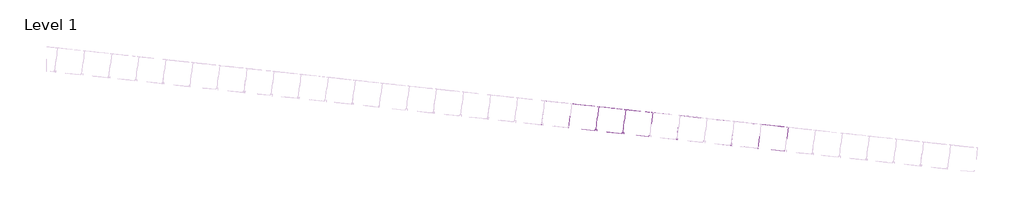
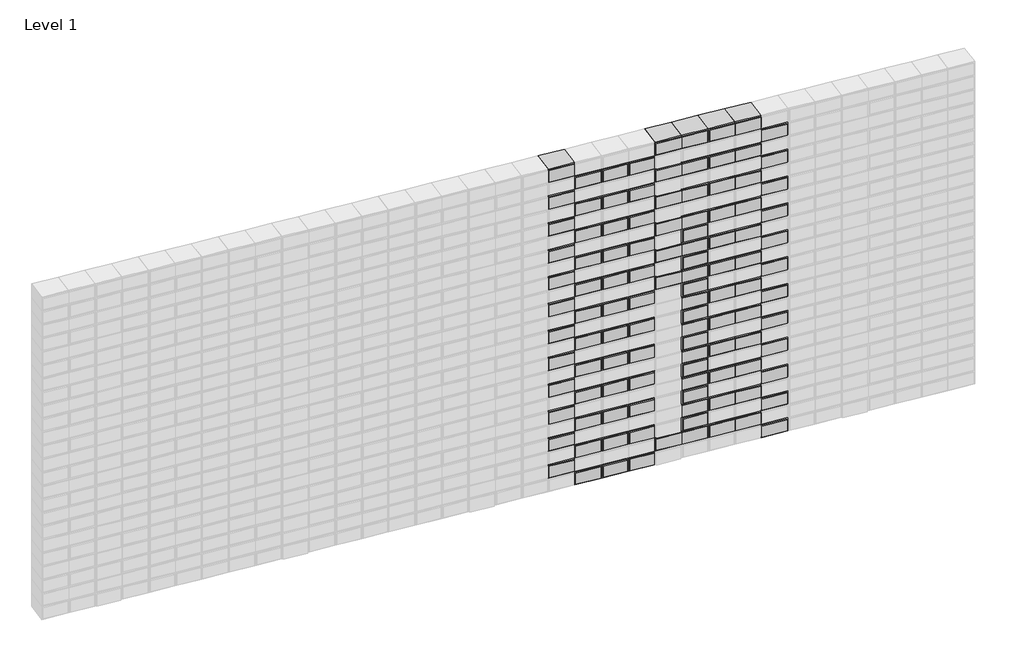
# One storey, part 16 of 18: 111 proxies.
"""IFC4 building model written with IfcOpenShell, lengths in millimetres."""

import ifcopenshell
import ifcopenshell.guid

model = None  # the IFC model being written
_history = None  # IfcOwnerHistory: only IFC2X3 demands one
_inside = {}  # id of a spatial element -> (the spatial element, [elements in it])
_under = {}  # id of a project, library or spatial element -> (it, [spatial elements below it])
_declared = {}  # id of a project -> (the project, [libraries it declares])
_typed = {}  # id of a type object -> (the type object, [elements of that type])
_made_of = {}  # id of a material, layer set ... -> (it, [elements and type objects made of it])


def new_model(schema):
    """Start an empty IFC model of exactly this schema.

    Asked for "IFC4X3", IfcOpenShell would pick the latest addendum, in which some entities
    have other attributes; the version numbers below select the first issue.
    IFC2X3 requires an IfcOwnerHistory on every rooted entity: one is made here for all.
    """
    global model, _history
    if schema == "IFC4X3":
        model = ifcopenshell.file(schema_version=(4, 3, 0, 0))
    else:
        model = ifcopenshell.file(schema=schema)
    _inside.clear()
    _under.clear()
    _declared.clear()
    _typed.clear()
    _made_of.clear()
    _history = None
    if model.schema == "IFC2X3":
        org = make("IfcOrganization", Name="unknown")
        user = make(
            "IfcPersonAndOrganization",
            ThePerson=make("IfcPerson", FamilyName="unknown"),
            TheOrganization=org,
        )
        app = make(
            "IfcApplication",
            ApplicationDeveloper=org,
            Version="unknown",
            ApplicationFullName="unknown",
            ApplicationIdentifier="unknown",
        )
        _history = make(
            "IfcOwnerHistory",
            OwningUser=user,
            OwningApplication=app,
            ChangeAction="ADDED",
            CreationDate=0,
        )
    return model


def make(cls, **values):
    """One entity of the class cls with the attributes given. An attribute that is None is left unset."""
    return model.create_entity(
        cls, **{name: value for name, value in values.items() if value is not None}
    )


def rooted(cls, **values):
    """An entity with a GlobalId (a new one), such as an element, a storey or a relation."""
    return make(cls, GlobalId=ifcopenshell.guid.new(), OwnerHistory=_history, **values)


def si_unit(unit_type, name, prefix=None):
    """IfcSIUnit, for example si_unit("LENGTHUNIT", "METRE", prefix="MILLI")."""
    return make("IfcSIUnit", UnitType=unit_type, Prefix=prefix, Name=name)


def assignment(units):
    """IfcUnitAssignment: the units of a project."""
    return None if units is None else make("IfcUnitAssignment", Units=units)


def point(xyz):
    """IfcCartesianPoint."""
    return None if xyz is None else make("IfcCartesianPoint", Coordinates=xyz)


def direction(xyz):
    """IfcDirection."""
    return None if xyz is None else make("IfcDirection", DirectionRatios=xyz)


def frame(location, z_axis=None, x_axis=None):
    """IfcAxis2Placement3D, a coordinate frame: its origin and axes. An axis left out is left unset."""
    return make(
        "IfcAxis2Placement3D",
        Location=point(location),
        Axis=direction(z_axis),
        RefDirection=direction(x_axis),
    )


def origin():
    """The frame at (0, 0, 0) with its axes left unset."""
    return frame((0.0, 0.0, 0.0))


def origin_with_axes():
    """The frame at (0, 0, 0) with the z axis (0, 0, 1) and the x axis (1, 0, 0) written out."""
    return frame((0.0, 0.0, 0.0), z_axis=(0.0, 0.0, 1.0), x_axis=(1.0, 0.0, 0.0))


def place(relative_to, where):
    """IfcLocalPlacement: puts the frame where relative to a parent placement (None: the world)."""
    return make(
        "IfcLocalPlacement", PlacementRelTo=relative_to, RelativePlacement=where
    )


def context(
    kind, dimensions, precision=None, world=None, true_north=None, identifier=None
):
    """IfcGeometricRepresentationContext, for example the 3D "Model" context."""
    return make(
        "IfcGeometricRepresentationContext",
        ContextIdentifier=identifier,
        ContextType=kind,
        CoordinateSpaceDimension=dimensions,
        Precision=precision,
        WorldCoordinateSystem=world,
        TrueNorth=true_north,
    )


def project(units=None, contexts=None):
    """IfcProject with its units and contexts."""
    return rooted(
        "IfcProject",
        Name="project",
        RepresentationContexts=contexts,
        UnitsInContext=assignment(units),
    )


def spatial(cls, under=None, at=None, **own):
    """A site, building, storey or space (cls), placed at a placement, below another one or the project."""
    s = rooted(cls, ObjectPlacement=at, **own)
    if under is not None:
        _under.setdefault(under.id(), (under, []))[1].append(s)
    return s


def polyline(points):
    """IfcPolyline through the points."""
    return make("IfcPolyline", Points=[point(p) for p in points])


def outline(outer, holes=None, kind="AREA"):
    """IfcArbitraryClosedProfileDef: a profile drawn as a closed curve; with holes, ...WithVoids."""
    if holes is None:
        return make("IfcArbitraryClosedProfileDef", ProfileType=kind, OuterCurve=outer)
    return make(
        "IfcArbitraryProfileDefWithVoids",
        ProfileType=kind,
        OuterCurve=outer,
        InnerCurves=holes,
    )


def extrude(swept, where, along, depth):
    """IfcExtrudedAreaSolid: the profile swept, set in the frame where, extruded along a direction by depth."""
    return make(
        "IfcExtrudedAreaSolid",
        SweptArea=swept,
        Position=where,
        ExtrudedDirection=direction(along),
        Depth=depth,
    )


def shape(context_of_items, identifier, shape_type, items):
    """IfcShapeRepresentation: the items that make up one representation, for example the "Body"."""
    return make(
        "IfcShapeRepresentation",
        ContextOfItems=context_of_items,
        RepresentationIdentifier=identifier,
        RepresentationType=shape_type,
        Items=items,
    )


def source(mapping_origin, context_of_items, identifier, shape_type, items):
    """IfcRepresentationMap: a shape defined once, which mapped items show again and again."""
    return make(
        "IfcRepresentationMap",
        MappingOrigin=mapping_origin,
        MappedRepresentation=shape(context_of_items, identifier, shape_type, items),
    )


def transform(
    local_origin,
    x_axis=None,
    y_axis=None,
    z_axis=None,
    scale=None,
    scale2=None,
    scale3=None,
    uniform=True,
):
    """IfcCartesianTransformationOperator3D, or its non-uniform kind. x_axis, y_axis, z_axis: its Axis1, 2, 3."""
    if uniform:
        return make(
            "IfcCartesianTransformationOperator3D",
            Axis1=direction(x_axis),
            Axis2=direction(y_axis),
            LocalOrigin=point(local_origin),
            Scale=scale,
            Axis3=direction(z_axis),
        )
    return make(
        "IfcCartesianTransformationOperator3DnonUniform",
        Axis1=direction(x_axis),
        Axis2=direction(y_axis),
        LocalOrigin=point(local_origin),
        Scale=scale,
        Axis3=direction(z_axis),
        Scale2=scale2,
        Scale3=scale3,
    )


def mapped(mapping_source, mapping_target):
    """IfcMappedItem: shows the shape of a source again, moved by a transform."""
    return make(
        "IfcMappedItem", MappingSource=mapping_source, MappingTarget=mapping_target
    )


def made_of(thing, what):
    """Note that an element or type object is made of a material, layer set ...; save() writes the relation."""
    if what is not None:
        _made_of.setdefault(what.id(), (what, []))[1].append(thing)
    return thing


def element(
    cls,
    number,
    at=None,
    inside=None,
    cuts=None,
    type_object=None,
    material=None,
    context=None,
    identifier="Body",
    shape_type=None,
    held_by="IfcProductDefinitionShape",
    body=None,
    shapes=None,
    **own,
):
    """One element of the class cls, such as IfcWall. Its Tag is "e" and its number.

    at: its placement. inside: the storey or other place that contains it. cuts: it is an
    opening in that element (IfcRelVoidsElement). A single representation is given by context,
    identifier, shape_type and body (its items); several are given by shapes. held_by: the class
    of the entity that holds the representations. save() writes the other relations.
    """
    e = rooted(cls, Tag="e%d" % number, ObjectPlacement=at, **own)
    if body is not None:
        shapes = [shape(context, identifier, shape_type, body)]
    if shapes is not None:
        e.Representation = make(held_by, Representations=shapes)
    if inside is not None:
        _inside.setdefault(inside.id(), (inside, []))[1].append(e)
    if cuts is not None:
        rooted(
            "IfcRelVoidsElement", RelatingBuildingElement=cuts, RelatedOpeningElement=e
        )
    if type_object is not None:
        _typed.setdefault(type_object.id(), (type_object, []))[1].append(e)
    return made_of(e, material)


def aggregate(whole, parts):
    """IfcRelAggregates: a whole, such as a stair, and the parts it consists of."""
    return rooted("IfcRelAggregates", RelatingObject=whole, RelatedObjects=parts)


def save(model, path):
    """Write the relations noted so far, then the file.

    IfcRelAggregates (storeys below a building ...), IfcRelContainedInSpatialStructure (elements
    in a storey), IfcRelDefinesByType, IfcRelAssociatesMaterial and IfcRelDeclares: one each for
    every whole, place, type object, material and project.
    """
    for whole, parts in _under.values():
        aggregate(whole, parts)
    for where, things in _inside.values():
        rooted(
            "IfcRelContainedInSpatialStructure",
            RelatedElements=things,
            RelatingStructure=where,
        )
    for kind, things in _typed.values():
        rooted("IfcRelDefinesByType", RelatedObjects=things, RelatingType=kind)
    for what, things in _made_of.values():
        rooted("IfcRelAssociatesMaterial", RelatedObjects=things, RelatingMaterial=what)
    for by, libraries in _declared.values():
        rooted("IfcRelDeclares", RelatingContext=by, RelatedDefinitions=libraries)
    model.write(path)


def geel_a5fc7152(model_context):
    return source(origin(), model_context, "Body", "SweptSolid", [
        extrude(outline(polyline([(131.1871262, 51.8695461), (24.8461542, 24.0369432), (23.5801491, 28.8740117), (125.0840527, 55.4406095), (111.9430518, 105.6488784), (10.4391482, 79.0822806), (9.1731432, 83.919349), (115.5141152, 111.7519519), (131.1871262, 51.8695461)])), origin_with_axes(), (0.0, 0.0, 1.0), 95.0),
        extrude(outline(polyline([(111.9430518, 105.6488784), (125.0840527, 55.4406095), (23.5801491, 28.8740117), (10.4391482, 79.0822806), (111.9430518, 105.6488784)])), origin_with_axes(), (0.0, 0.0, 1.0), 100.0),
    ])


def geel_ff5a4212(model_context):
    return source(origin(), model_context, "Body", "SweptSolid", [
        extrude(outline(polyline([(24.8461542, 24.0369432), (9.1731432, 83.919349), (115.5141152, 111.7519519), (116.7801202, 106.9148835), (15.2762167, 80.3482856), (28.4172176, 30.1400167), (129.9211211, 56.7066146), (131.1871262, 51.8695461), (24.8461542, 24.0369432)])), origin_with_axes(), (0.0, 0.0, 1.0), 95.0),
        extrude(outline(polyline([(116.7801202, 106.9148835), (129.9211211, 56.7066146), (28.4172176, 30.1400167), (15.2762167, 80.3482856), (116.7801202, 106.9148835)])), origin_with_axes(), (0.0, 0.0, 1.0), 100.0),
    ])


def rood_14a66368(model_context):
    return source(origin(), model_context, "Body", "SweptSolid", [
        extrude(outline(polyline([(24.8461542, 24.0369432), (9.1731432, 83.919349), (115.5141152, 111.7519519), (131.1871262, 51.8695461), (24.8461542, 24.0369432)]), holes=[polyline([(125.0840527, 55.4406095), (111.9430518, 105.6488784), (15.2762167, 80.3482856), (28.4172176, 30.1400167), (125.0840527, 55.4406095)])]), origin_with_axes(), (0.0, 0.0, 1.0), 95.0),
        extrude(outline(polyline([(111.9430518, 105.6488784), (125.0840527, 55.4406095), (28.4172176, 30.1400167), (15.2762167, 80.3482856), (111.9430518, 105.6488784)])), origin_with_axes(), (0.0, 0.0, 1.0), 100.0),
    ])


model = new_model("IFC4")

# Units and contexts
model_context = context("Model", 3, world=origin())
ifc_project = project(units=[si_unit("LENGTHUNIT", "METRE", prefix="MILLI")], contexts=[model_context])

# Site, building, storey
site = spatial("IfcSite", under=ifc_project)
building = spatial("IfcBuilding", under=site)
storey = spatial("IfcBuildingStorey", under=building, Name="Level 1", Elevation=0.0)

# Proxies
placement = place(None, origin())
geel_shape = geel_a5fc7152(model_context)
element("IfcBuildingElementProxy", 1, Name="Geel", ObjectType="Geel", at=placement, inside=storey, context=model_context, shape_type="MappedRepresentation", body=[
    mapped(geel_shape, transform((11609.0111995, -4573.7784941, 2168.7358475), x_axis=(0.9617275503729374, -0.1047347566147725, -0.25320100633787673), y_axis=(0.25171277368869216, -0.02741220845642974, 0.9674136914420255), z_axis=(-0.10826263628609081, -0.9941223272738551, 0.0))),
])
element("IfcBuildingElementProxy", 2, Name="Geel", ObjectType="Geel", at=placement, inside=storey, context=model_context, shape_type="MappedRepresentation", body=[
    mapped(geel_shape, transform((11609.0111995, -4573.7784941, 2292.5348104), x_axis=(0.9617275503729374, -0.1047347566147725, -0.25320100633787673), y_axis=(0.25171277368869216, -0.02741220845642974, 0.9674136914420255), z_axis=(-0.10826263628609081, -0.9941223272738551, 0.0))),
])
element("IfcBuildingElementProxy", 3, Name="Geel", ObjectType="Geel", at=placement, inside=storey, context=model_context, shape_type="MappedRepresentation", body=[
    mapped(geel_shape, transform((11609.0111995, -4573.7784941, 2416.3337732), x_axis=(0.9617275503729384, -0.1047347566147726, -0.25320100633787307), y_axis=(0.25171277368868855, -0.02741220845642934, 0.9674136914420265), z_axis=(-0.10826263628609081, -0.994122327273855, 0.0))),
])
element("IfcBuildingElementProxy", 4, Name="Geel", ObjectType="Geel", at=placement, inside=storey, context=model_context, shape_type="MappedRepresentation", body=[
    mapped(geel_shape, transform((11609.0111995, -4573.7784941, 2540.132736), x_axis=(0.9617275503729374, -0.1047347566147725, -0.25320100633787673), y_axis=(0.25171277368869216, -0.02741220845642974, 0.9674136914420255), z_axis=(-0.10826263628609081, -0.9941223272738551, 0.0))),
])
element("IfcBuildingElementProxy", 5, Name="Geel", ObjectType="Geel", at=placement, inside=storey, context=model_context, shape_type="MappedRepresentation", body=[
    mapped(geel_shape, transform((11609.0111995, -4573.7784941, 2663.9316989), x_axis=(0.9617275503729374, -0.1047347566147725, -0.25320100633787673), y_axis=(0.25171277368869216, -0.02741220845642974, 0.9674136914420255), z_axis=(-0.10826263628609081, -0.9941223272738551, 0.0))),
])
element("IfcBuildingElementProxy", 6, Name="Geel", ObjectType="Geel", at=placement, inside=storey, context=model_context, shape_type="MappedRepresentation", body=[
    mapped(geel_shape, transform((11609.0111995, -4573.7784941, 2787.7306617), x_axis=(0.9617275503729374, -0.1047347566147725, -0.25320100633787673), y_axis=(0.25171277368869216, -0.02741220845642974, 0.9674136914420255), z_axis=(-0.10826263628609081, -0.9941223272738551, 0.0))),
])
element("IfcBuildingElementProxy", 7, Name="Geel", ObjectType="Geel", at=placement, inside=storey, context=model_context, shape_type="MappedRepresentation", body=[
    mapped(geel_shape, transform((11609.0111995, -4573.7784941, 2911.5296245), x_axis=(0.9617275503729374, -0.1047347566147725, -0.25320100633787673), y_axis=(0.25171277368869216, -0.02741220845642974, 0.9674136914420255), z_axis=(-0.10826263628609081, -0.9941223272738551, 0.0))),
])
element("IfcBuildingElementProxy", 8, Name="Geel", ObjectType="Geel", at=placement, inside=storey, context=model_context, shape_type="MappedRepresentation", body=[
    mapped(geel_shape, transform((11609.0111995, -4573.7784941, 3035.3285874), x_axis=(0.9617275503729374, -0.1047347566147725, -0.25320100633787673), y_axis=(0.25171277368869216, -0.02741220845642974, 0.9674136914420255), z_axis=(-0.10826263628609081, -0.9941223272738551, 0.0))),
])
element("IfcBuildingElementProxy", 9, Name="Geel", ObjectType="Geel", at=placement, inside=storey, context=model_context, shape_type="MappedRepresentation", body=[
    mapped(geel_shape, transform((11609.0111995, -4573.7784941, 3159.1275502), x_axis=(0.9617275503729374, -0.1047347566147725, -0.25320100633787673), y_axis=(0.25171277368869216, -0.02741220845642974, 0.9674136914420255), z_axis=(-0.10826263628609081, -0.9941223272738551, 0.0))),
])
element("IfcBuildingElementProxy", 10, Name="Geel", ObjectType="Geel", at=placement, inside=storey, context=model_context, shape_type="MappedRepresentation", body=[
    mapped(geel_shape, transform((11609.0111995, -4573.7784941, 3282.926513), x_axis=(0.9617275503729374, -0.1047347566147725, -0.25320100633787673), y_axis=(0.25171277368869216, -0.02741220845642974, 0.9674136914420255), z_axis=(-0.10826263628609081, -0.9941223272738551, 0.0))),
])
element("IfcBuildingElementProxy", 11, Name="Geel", ObjectType="Geel", at=placement, inside=storey, context=model_context, shape_type="MappedRepresentation", body=[
    mapped(geel_shape, transform((11609.0111995, -4573.7784941, 3406.7254759), x_axis=(0.9617275503729374, -0.1047347566147725, -0.25320100633787673), y_axis=(0.25171277368869216, -0.02741220845642974, 0.9674136914420255), z_axis=(-0.10826263628609081, -0.9941223272738551, 0.0))),
])
element("IfcBuildingElementProxy", 12, Name="Geel", ObjectType="Geel", at=placement, inside=storey, context=model_context, shape_type="MappedRepresentation", body=[
    mapped(geel_shape, transform((11609.0111995, -4573.7784941, 2044.9368847), x_axis=(0.9617275503729384, -0.1047347566147726, -0.25320100633787307), y_axis=(0.25171277368868855, -0.02741220845642934, 0.9674136914420265), z_axis=(-0.10826263628609081, -0.994122327273855, 0.0))),
])
element("IfcBuildingElementProxy", 13, Name="Geel", ObjectType="Geel", at=placement, inside=storey, context=model_context, shape_type="MappedRepresentation", body=[
    mapped(geel_shape, transform((11062.6268786, -4514.2757494, 2168.7358475), x_axis=(0.9617275503729374, -0.1047347566147725, -0.25320100633787673), y_axis=(0.25171277368869216, -0.02741220845642974, 0.9674136914420255), z_axis=(-0.10826263628609081, -0.9941223272738551, 0.0))),
])
element("IfcBuildingElementProxy", 14, Name="Geel", ObjectType="Geel", at=placement, inside=storey, context=model_context, shape_type="MappedRepresentation", body=[
    mapped(geel_shape, transform((11827.5649279, -4597.579592, 2168.7358475), x_axis=(0.9617275503729414, -0.10473475661477494, -0.25320100633786047), y_axis=(0.251712773688676, -0.027412208456428513, 0.9674136914420297), z_axis=(-0.10826263628609288, -0.9941223272738549, 0.0))),
])
element("IfcBuildingElementProxy", 15, Name="Geel", ObjectType="Geel", at=placement, inside=storey, context=model_context, shape_type="MappedRepresentation", body=[
    mapped(geel_shape, transform((11062.6268786, -4514.2757494, 2292.5348104), x_axis=(0.9617275503729374, -0.1047347566147725, -0.25320100633787673), y_axis=(0.25171277368869216, -0.02741220845642974, 0.9674136914420255), z_axis=(-0.10826263628609081, -0.9941223272738551, 0.0))),
])
element("IfcBuildingElementProxy", 16, Name="Geel", ObjectType="Geel", at=placement, inside=storey, context=model_context, shape_type="MappedRepresentation", body=[
    mapped(geel_shape, transform((11827.5649279, -4597.579592, 2292.5348104), x_axis=(0.9617275503729414, -0.10473475661477494, -0.25320100633786047), y_axis=(0.251712773688676, -0.027412208456428513, 0.9674136914420297), z_axis=(-0.10826263628609288, -0.9941223272738549, 0.0))),
])
element("IfcBuildingElementProxy", 17, Name="Geel", ObjectType="Geel", at=placement, inside=storey, context=model_context, shape_type="MappedRepresentation", body=[
    mapped(geel_shape, transform((11062.6268786, -4514.2757494, 2416.3337732), x_axis=(0.9617275503729384, -0.1047347566147726, -0.25320100633787307), y_axis=(0.25171277368868855, -0.02741220845642934, 0.9674136914420265), z_axis=(-0.10826263628609081, -0.994122327273855, 0.0))),
])
element("IfcBuildingElementProxy", 18, Name="Geel", ObjectType="Geel", at=placement, inside=storey, context=model_context, shape_type="MappedRepresentation", body=[
    mapped(geel_shape, transform((11827.5649279, -4597.579592, 2416.3337732), x_axis=(0.9617275503729424, -0.10473475661477503, -0.25320100633785697), y_axis=(0.25171277368867234, -0.027412208456428104, 0.9674136914420307), z_axis=(-0.10826263628609285, -0.9941223272738547, 0.0))),
])
element("IfcBuildingElementProxy", 19, Name="Geel", ObjectType="Geel", at=placement, inside=storey, context=model_context, shape_type="MappedRepresentation", body=[
    mapped(geel_shape, transform((11062.6268786, -4514.2757494, 2540.132736), x_axis=(0.9617275503729374, -0.1047347566147725, -0.25320100633787673), y_axis=(0.25171277368869216, -0.02741220845642974, 0.9674136914420255), z_axis=(-0.10826263628609081, -0.9941223272738551, 0.0))),
])
element("IfcBuildingElementProxy", 20, Name="Geel", ObjectType="Geel", at=placement, inside=storey, context=model_context, shape_type="MappedRepresentation", body=[
    mapped(geel_shape, transform((11827.5649279, -4597.579592, 2540.132736), x_axis=(0.9617275503729414, -0.10473475661477494, -0.25320100633786047), y_axis=(0.251712773688676, -0.027412208456428513, 0.9674136914420297), z_axis=(-0.10826263628609288, -0.9941223272738549, 0.0))),
])
element("IfcBuildingElementProxy", 21, Name="Geel", ObjectType="Geel", at=placement, inside=storey, context=model_context, shape_type="MappedRepresentation", body=[
    mapped(geel_shape, transform((11062.6268786, -4514.2757494, 2663.9316989), x_axis=(0.9617275503729374, -0.1047347566147725, -0.25320100633787673), y_axis=(0.25171277368869216, -0.02741220845642974, 0.9674136914420255), z_axis=(-0.10826263628609081, -0.9941223272738551, 0.0))),
])
element("IfcBuildingElementProxy", 22, Name="Geel", ObjectType="Geel", at=placement, inside=storey, context=model_context, shape_type="MappedRepresentation", body=[
    mapped(geel_shape, transform((11827.5649279, -4597.579592, 2663.9316989), x_axis=(0.9617275503729414, -0.10473475661477494, -0.25320100633786047), y_axis=(0.251712773688676, -0.027412208456428513, 0.9674136914420297), z_axis=(-0.10826263628609288, -0.9941223272738549, 0.0))),
])
element("IfcBuildingElementProxy", 23, Name="Geel", ObjectType="Geel", at=placement, inside=storey, context=model_context, shape_type="MappedRepresentation", body=[
    mapped(geel_shape, transform((11062.6268786, -4514.2757494, 2787.7306617), x_axis=(0.9617275503729374, -0.1047347566147725, -0.25320100633787673), y_axis=(0.25171277368869216, -0.02741220845642974, 0.9674136914420255), z_axis=(-0.10826263628609081, -0.9941223272738551, 0.0))),
])
element("IfcBuildingElementProxy", 24, Name="Geel", ObjectType="Geel", at=placement, inside=storey, context=model_context, shape_type="MappedRepresentation", body=[
    mapped(geel_shape, transform((11827.5649279, -4597.579592, 2787.7306617), x_axis=(0.9617275503729414, -0.10473475661477494, -0.25320100633786047), y_axis=(0.251712773688676, -0.027412208456428513, 0.9674136914420297), z_axis=(-0.10826263628609288, -0.9941223272738549, 0.0))),
])
element("IfcBuildingElementProxy", 25, Name="Geel", ObjectType="Geel", at=placement, inside=storey, context=model_context, shape_type="MappedRepresentation", body=[
    mapped(geel_shape, transform((11062.6268786, -4514.2757494, 2911.5296245), x_axis=(0.9617275503729374, -0.1047347566147725, -0.25320100633787673), y_axis=(0.25171277368869216, -0.02741220845642974, 0.9674136914420255), z_axis=(-0.10826263628609081, -0.9941223272738551, 0.0))),
])
element("IfcBuildingElementProxy", 26, Name="Geel", ObjectType="Geel", at=placement, inside=storey, context=model_context, shape_type="MappedRepresentation", body=[
    mapped(geel_shape, transform((11827.5649279, -4597.579592, 2911.5296245), x_axis=(0.9617275503729414, -0.10473475661477494, -0.25320100633786047), y_axis=(0.251712773688676, -0.027412208456428513, 0.9674136914420297), z_axis=(-0.10826263628609288, -0.9941223272738549, 0.0))),
])
element("IfcBuildingElementProxy", 27, Name="Geel", ObjectType="Geel", at=placement, inside=storey, context=model_context, shape_type="MappedRepresentation", body=[
    mapped(geel_shape, transform((11062.6268786, -4514.2757494, 3035.3285874), x_axis=(0.9617275503729374, -0.1047347566147725, -0.25320100633787673), y_axis=(0.25171277368869216, -0.02741220845642974, 0.9674136914420255), z_axis=(-0.10826263628609081, -0.9941223272738551, 0.0))),
])
element("IfcBuildingElementProxy", 28, Name="Geel", ObjectType="Geel", at=placement, inside=storey, context=model_context, shape_type="MappedRepresentation", body=[
    mapped(geel_shape, transform((11827.5649279, -4597.579592, 3035.3285874), x_axis=(0.9617275503729414, -0.10473475661477494, -0.25320100633786047), y_axis=(0.251712773688676, -0.027412208456428513, 0.9674136914420297), z_axis=(-0.10826263628609288, -0.9941223272738549, 0.0))),
])
element("IfcBuildingElementProxy", 29, Name="Geel", ObjectType="Geel", at=placement, inside=storey, context=model_context, shape_type="MappedRepresentation", body=[
    mapped(geel_shape, transform((11062.6268786, -4514.2757494, 3159.1275502), x_axis=(0.9617275503729374, -0.1047347566147725, -0.25320100633787673), y_axis=(0.25171277368869216, -0.02741220845642974, 0.9674136914420255), z_axis=(-0.10826263628609081, -0.9941223272738551, 0.0))),
])
element("IfcBuildingElementProxy", 30, Name="Geel", ObjectType="Geel", at=placement, inside=storey, context=model_context, shape_type="MappedRepresentation", body=[
    mapped(geel_shape, transform((11827.5649279, -4597.579592, 3159.1275502), x_axis=(0.9617275503729414, -0.10473475661477494, -0.25320100633786047), y_axis=(0.251712773688676, -0.027412208456428513, 0.9674136914420297), z_axis=(-0.10826263628609288, -0.9941223272738549, 0.0))),
])
element("IfcBuildingElementProxy", 31, Name="Geel", ObjectType="Geel", at=placement, inside=storey, context=model_context, shape_type="MappedRepresentation", body=[
    mapped(geel_shape, transform((11062.6268786, -4514.2757494, 3282.926513), x_axis=(0.9617275503729374, -0.1047347566147725, -0.25320100633787673), y_axis=(0.25171277368869216, -0.02741220845642974, 0.9674136914420255), z_axis=(-0.10826263628609081, -0.9941223272738551, 0.0))),
])
element("IfcBuildingElementProxy", 32, Name="Geel", ObjectType="Geel", at=placement, inside=storey, context=model_context, shape_type="MappedRepresentation", body=[
    mapped(geel_shape, transform((11827.5649279, -4597.579592, 3282.926513), x_axis=(0.9617275503729414, -0.10473475661477494, -0.25320100633786047), y_axis=(0.251712773688676, -0.027412208456428513, 0.9674136914420297), z_axis=(-0.10826263628609288, -0.9941223272738549, 0.0))),
])
element("IfcBuildingElementProxy", 33, Name="Geel", ObjectType="Geel", at=placement, inside=storey, context=model_context, shape_type="MappedRepresentation", body=[
    mapped(geel_shape, transform((11062.6268786, -4514.2757494, 3406.7254759), x_axis=(0.9617275503729374, -0.1047347566147725, -0.25320100633787673), y_axis=(0.25171277368869216, -0.02741220845642974, 0.9674136914420255), z_axis=(-0.10826263628609081, -0.9941223272738551, 0.0))),
])
element("IfcBuildingElementProxy", 34, Name="Geel", ObjectType="Geel", at=placement, inside=storey, context=model_context, shape_type="MappedRepresentation", body=[
    mapped(geel_shape, transform((11827.5649279, -4597.579592, 3406.7254759), x_axis=(0.9617275503729414, -0.10473475661477494, -0.25320100633786047), y_axis=(0.251712773688676, -0.027412208456428513, 0.9674136914420297), z_axis=(-0.10826263628609288, -0.9941223272738549, 0.0))),
])
element("IfcBuildingElementProxy", 35, Name="Geel", ObjectType="Geel", at=placement, inside=storey, context=model_context, shape_type="MappedRepresentation", body=[
    mapped(geel_shape, transform((11062.6268786, -4514.2757494, 2044.9368847), x_axis=(0.9617275503729384, -0.1047347566147726, -0.25320100633787307), y_axis=(0.25171277368868855, -0.02741220845642934, 0.9674136914420265), z_axis=(-0.10826263628609081, -0.994122327273855, 0.0))),
])
element("IfcBuildingElementProxy", 36, Name="Geel", ObjectType="Geel", at=placement, inside=storey, context=model_context, shape_type="MappedRepresentation", body=[
    mapped(geel_shape, transform((11827.5649279, -4597.579592, 2044.9368847), x_axis=(0.9617275503729424, -0.10473475661477503, -0.25320100633785697), y_axis=(0.25171277368867234, -0.027412208456428104, 0.9674136914420307), z_axis=(-0.10826263628609285, -0.9941223272738547, 0.0))),
])
geel_2_shape = geel_ff5a4212(model_context)
element("IfcBuildingElementProxy", 37, Name="Geel", ObjectType="Geel", at=placement, inside=storey, context=model_context, shape_type="MappedRepresentation", body=[
    mapped(geel_2_shape, transform((11499.7343354, -4561.8779452, 2787.7306617), x_axis=(0.9617275503729381, -0.10473475661476775, -0.25320100633787634), y_axis=(0.2517127736886919, -0.02741220845642843, 0.9674136914420257), z_axis=(-0.1082626362860859, -0.9941223272738555, 0.0))),
])
element("IfcBuildingElementProxy", 38, Name="Geel", ObjectType="Geel", at=placement, inside=storey, context=model_context, shape_type="MappedRepresentation", body=[
    mapped(geel_2_shape, transform((11499.7343354, -4561.8779452, 2911.5296245), x_axis=(0.9617275503729381, -0.10473475661476775, -0.25320100633787634), y_axis=(0.2517127736886919, -0.02741220845642843, 0.9674136914420257), z_axis=(-0.1082626362860859, -0.9941223272738555, 0.0))),
])
element("IfcBuildingElementProxy", 39, Name="Geel", ObjectType="Geel", at=placement, inside=storey, context=model_context, shape_type="MappedRepresentation", body=[
    mapped(geel_2_shape, transform((11499.7343354, -4561.8779452, 3035.3285874), x_axis=(0.9617275503729381, -0.10473475661476775, -0.25320100633787634), y_axis=(0.2517127736886919, -0.02741220845642843, 0.9674136914420257), z_axis=(-0.1082626362860859, -0.9941223272738555, 0.0))),
])
element("IfcBuildingElementProxy", 40, Name="Geel", ObjectType="Geel", at=placement, inside=storey, context=model_context, shape_type="MappedRepresentation", body=[
    mapped(geel_2_shape, transform((11499.7343354, -4561.8779452, 3159.1275502), x_axis=(0.9617275503729381, -0.10473475661476775, -0.25320100633787634), y_axis=(0.2517127736886919, -0.02741220845642843, 0.9674136914420257), z_axis=(-0.1082626362860859, -0.9941223272738555, 0.0))),
])
element("IfcBuildingElementProxy", 41, Name="Geel", ObjectType="Geel", at=placement, inside=storey, context=model_context, shape_type="MappedRepresentation", body=[
    mapped(geel_2_shape, transform((11499.7343354, -4561.8779452, 3282.926513), x_axis=(0.9617275503729381, -0.10473475661476775, -0.25320100633787634), y_axis=(0.2517127736886919, -0.02741220845642843, 0.9674136914420257), z_axis=(-0.1082626362860859, -0.9941223272738555, 0.0))),
])
element("IfcBuildingElementProxy", 42, Name="Geel", ObjectType="Geel", at=placement, inside=storey, context=model_context, shape_type="MappedRepresentation", body=[
    mapped(geel_2_shape, transform((11499.7343354, -4561.8779452, 3406.7254759), x_axis=(0.9617275503729381, -0.10473475661476775, -0.25320100633787634), y_axis=(0.2517127736886919, -0.02741220845642843, 0.9674136914420257), z_axis=(-0.1082626362860859, -0.9941223272738555, 0.0))),
])
element("IfcBuildingElementProxy", 43, Name="Geel", ObjectType="Geel", at=placement, inside=storey, context=model_context, shape_type="MappedRepresentation", body=[
    mapped(geel_2_shape, transform((11499.7343354, -4561.8779452, 2044.9368847), x_axis=(0.961727550372939, -0.10473475661476785, -0.2532010063378727), y_axis=(0.2517127736886882, -0.02741220845642804, 0.9674136914420266), z_axis=(-0.1082626362860859, -0.9941223272738555, 0.0))),
])
element("IfcBuildingElementProxy", 44, Name="Geel", ObjectType="Geel", at=placement, inside=storey, context=model_context, shape_type="MappedRepresentation", body=[
    mapped(geel_2_shape, transform((11718.2880637, -4585.679043, 2168.7358475), x_axis=(0.9617275503729374, -0.1047347566147725, -0.25320100633787673), y_axis=(0.25171277368869216, -0.02741220845642974, 0.9674136914420255), z_axis=(-0.10826263628609081, -0.9941223272738551, 0.0))),
])
element("IfcBuildingElementProxy", 45, Name="Geel", ObjectType="Geel", at=placement, inside=storey, context=model_context, shape_type="MappedRepresentation", body=[
    mapped(geel_2_shape, transform((11718.2880637, -4585.679043, 2292.5348104), x_axis=(0.9617275503729374, -0.1047347566147725, -0.25320100633787673), y_axis=(0.25171277368869216, -0.02741220845642974, 0.9674136914420255), z_axis=(-0.10826263628609081, -0.9941223272738551, 0.0))),
])
element("IfcBuildingElementProxy", 46, Name="Geel", ObjectType="Geel", at=placement, inside=storey, context=model_context, shape_type="MappedRepresentation", body=[
    mapped(geel_2_shape, transform((11718.2880637, -4585.679043, 2416.3337732), x_axis=(0.9617275503729384, -0.1047347566147726, -0.25320100633787307), y_axis=(0.25171277368868855, -0.02741220845642934, 0.9674136914420265), z_axis=(-0.10826263628609081, -0.994122327273855, 0.0))),
])
element("IfcBuildingElementProxy", 47, Name="Geel", ObjectType="Geel", at=placement, inside=storey, context=model_context, shape_type="MappedRepresentation", body=[
    mapped(geel_2_shape, transform((11718.2880637, -4585.679043, 2540.132736), x_axis=(0.9617275503729374, -0.1047347566147725, -0.25320100633787673), y_axis=(0.25171277368869216, -0.02741220845642974, 0.9674136914420255), z_axis=(-0.10826263628609081, -0.9941223272738551, 0.0))),
])
element("IfcBuildingElementProxy", 48, Name="Geel", ObjectType="Geel", at=placement, inside=storey, context=model_context, shape_type="MappedRepresentation", body=[
    mapped(geel_2_shape, transform((11718.2880637, -4585.679043, 2663.9316989), x_axis=(0.9617275503729374, -0.1047347566147725, -0.25320100633787673), y_axis=(0.25171277368869216, -0.02741220845642974, 0.9674136914420255), z_axis=(-0.10826263628609081, -0.9941223272738551, 0.0))),
])
element("IfcBuildingElementProxy", 49, Name="Geel", ObjectType="Geel", at=placement, inside=storey, context=model_context, shape_type="MappedRepresentation", body=[
    mapped(geel_2_shape, transform((11718.2880637, -4585.679043, 2787.7306617), x_axis=(0.9617275503729374, -0.1047347566147725, -0.25320100633787673), y_axis=(0.25171277368869216, -0.02741220845642974, 0.9674136914420255), z_axis=(-0.10826263628609081, -0.9941223272738551, 0.0))),
])
element("IfcBuildingElementProxy", 50, Name="Geel", ObjectType="Geel", at=placement, inside=storey, context=model_context, shape_type="MappedRepresentation", body=[
    mapped(geel_2_shape, transform((11718.2880637, -4585.679043, 2911.5296245), x_axis=(0.9617275503729374, -0.1047347566147725, -0.25320100633787673), y_axis=(0.25171277368869216, -0.02741220845642974, 0.9674136914420255), z_axis=(-0.10826263628609081, -0.9941223272738551, 0.0))),
])
element("IfcBuildingElementProxy", 51, Name="Geel", ObjectType="Geel", at=placement, inside=storey, context=model_context, shape_type="MappedRepresentation", body=[
    mapped(geel_2_shape, transform((11718.2880637, -4585.679043, 3035.3285874), x_axis=(0.9617275503729374, -0.1047347566147725, -0.25320100633787673), y_axis=(0.25171277368869216, -0.02741220845642974, 0.9674136914420255), z_axis=(-0.10826263628609081, -0.9941223272738551, 0.0))),
])
element("IfcBuildingElementProxy", 52, Name="Geel", ObjectType="Geel", at=placement, inside=storey, context=model_context, shape_type="MappedRepresentation", body=[
    mapped(geel_2_shape, transform((11718.2880637, -4585.679043, 3159.1275502), x_axis=(0.9617275503729374, -0.1047347566147725, -0.25320100633787673), y_axis=(0.25171277368869216, -0.02741220845642974, 0.9674136914420255), z_axis=(-0.10826263628609081, -0.9941223272738551, 0.0))),
])
element("IfcBuildingElementProxy", 53, Name="Geel", ObjectType="Geel", at=placement, inside=storey, context=model_context, shape_type="MappedRepresentation", body=[
    mapped(geel_2_shape, transform((11718.2880637, -4585.679043, 3282.926513), x_axis=(0.9617275503729374, -0.1047347566147725, -0.25320100633787673), y_axis=(0.25171277368869216, -0.02741220845642974, 0.9674136914420255), z_axis=(-0.10826263628609081, -0.9941223272738551, 0.0))),
])
element("IfcBuildingElementProxy", 54, Name="Geel", ObjectType="Geel", at=placement, inside=storey, context=model_context, shape_type="MappedRepresentation", body=[
    mapped(geel_2_shape, transform((11718.2880637, -4585.679043, 3406.7254759), x_axis=(0.9617275503729374, -0.1047347566147725, -0.25320100633787673), y_axis=(0.25171277368869216, -0.02741220845642974, 0.9674136914420255), z_axis=(-0.10826263628609081, -0.9941223272738551, 0.0))),
])
element("IfcBuildingElementProxy", 55, Name="Geel", ObjectType="Geel", at=placement, inside=storey, context=model_context, shape_type="MappedRepresentation", body=[
    mapped(geel_2_shape, transform((11718.2880637, -4585.679043, 2044.9368847), x_axis=(0.9617275503729384, -0.1047347566147726, -0.25320100633787307), y_axis=(0.25171277368868855, -0.02741220845642934, 0.9674136914420265), z_axis=(-0.10826263628609081, -0.994122327273855, 0.0))),
])
element("IfcBuildingElementProxy", 56, Name="Rood", ObjectType="Rood", at=placement, inside=storey, context=model_context, shape_type="MappedRepresentation", body=[
    mapped(geel_shape, transform((11171.9037428, -4526.1762984, 2106.8363661), x_axis=(0.9617275503729374, -0.1047347566147725, -0.25320100633787673), y_axis=(0.25171277368869216, -0.02741220845642974, 0.9674136914420255), z_axis=(-0.10826263628609081, -0.9941223272738551, 0.0))),
])
element("IfcBuildingElementProxy", 57, Name="Rood", ObjectType="Rood", at=placement, inside=storey, context=model_context, shape_type="MappedRepresentation", body=[
    mapped(geel_shape, transform((11936.8417921, -4609.4801409, 2106.8363661), x_axis=(0.9617275503729374, -0.10473475661477244, -0.25320100633787673), y_axis=(0.25171277368869216, -0.027412208456429728, 0.9674136914420255), z_axis=(-0.10826263628609079, -0.9941223272738551, 0.0))),
])
element("IfcBuildingElementProxy", 58, Name="Rood", ObjectType="Rood", at=placement, inside=storey, context=model_context, shape_type="MappedRepresentation", body=[
    mapped(geel_shape, transform((11171.9037428, -4526.1762984, 2230.6353289), x_axis=(0.9617275503729384, -0.1047347566147726, -0.25320100633787307), y_axis=(0.25171277368868855, -0.02741220845642934, 0.9674136914420265), z_axis=(-0.10826263628609081, -0.994122327273855, 0.0))),
])
element("IfcBuildingElementProxy", 59, Name="Rood", ObjectType="Rood", at=placement, inside=storey, context=model_context, shape_type="MappedRepresentation", body=[
    mapped(geel_shape, transform((11936.8417921, -4609.4801409, 2230.6353289), x_axis=(0.9617275503729384, -0.10473475661477255, -0.25320100633787307), y_axis=(0.25171277368868855, -0.027412208456429325, 0.9674136914420265), z_axis=(-0.10826263628609077, -0.994122327273855, 0.0))),
])
element("IfcBuildingElementProxy", 60, Name="Rood", ObjectType="Rood", at=placement, inside=storey, context=model_context, shape_type="MappedRepresentation", body=[
    mapped(geel_shape, transform((11171.9037428, -4526.1762984, 2354.4342918), x_axis=(0.9617275503729374, -0.1047347566147725, -0.25320100633787673), y_axis=(0.25171277368869216, -0.02741220845642974, 0.9674136914420255), z_axis=(-0.10826263628609081, -0.9941223272738551, 0.0))),
])
element("IfcBuildingElementProxy", 61, Name="Rood", ObjectType="Rood", at=placement, inside=storey, context=model_context, shape_type="MappedRepresentation", body=[
    mapped(geel_shape, transform((11936.8417921, -4609.4801409, 2354.4342918), x_axis=(0.9617275503729374, -0.10473475661477244, -0.25320100633787673), y_axis=(0.25171277368869216, -0.027412208456429728, 0.9674136914420255), z_axis=(-0.10826263628609079, -0.9941223272738551, 0.0))),
])
element("IfcBuildingElementProxy", 62, Name="Rood", ObjectType="Rood", at=placement, inside=storey, context=model_context, shape_type="MappedRepresentation", body=[
    mapped(geel_shape, transform((11171.9037428, -4526.1762984, 2478.2332546), x_axis=(0.9617275503729374, -0.1047347566147725, -0.25320100633787673), y_axis=(0.25171277368869216, -0.02741220845642974, 0.9674136914420255), z_axis=(-0.10826263628609081, -0.9941223272738551, 0.0))),
])
element("IfcBuildingElementProxy", 63, Name="Rood", ObjectType="Rood", at=placement, inside=storey, context=model_context, shape_type="MappedRepresentation", body=[
    mapped(geel_shape, transform((11936.8417921, -4609.4801409, 2478.2332546), x_axis=(0.9617275503729374, -0.10473475661477244, -0.25320100633787673), y_axis=(0.25171277368869216, -0.027412208456429728, 0.9674136914420255), z_axis=(-0.10826263628609079, -0.9941223272738551, 0.0))),
])
element("IfcBuildingElementProxy", 64, Name="Rood", ObjectType="Rood", at=placement, inside=storey, context=model_context, shape_type="MappedRepresentation", body=[
    mapped(geel_shape, transform((11171.9037428, -4526.1762984, 2602.0322174), x_axis=(0.9617275503729394, -0.10473475661477268, -0.2532010063378695), y_axis=(0.2517127736886849, -0.027412208456428923, 0.9674136914420275), z_axis=(-0.1082626362860908, -0.9941223272738551, 0.0))),
])
element("IfcBuildingElementProxy", 65, Name="Rood", ObjectType="Rood", at=placement, inside=storey, context=model_context, shape_type="MappedRepresentation", body=[
    mapped(geel_shape, transform((11936.8417921, -4609.4801409, 2602.0322174), x_axis=(0.9617275503729394, -0.10473475661477262, -0.2532010063378695), y_axis=(0.2517127736886849, -0.027412208456428916, 0.9674136914420275), z_axis=(-0.10826263628609076, -0.9941223272738551, 0.0))),
])
element("IfcBuildingElementProxy", 66, Name="Rood", ObjectType="Rood", at=placement, inside=storey, context=model_context, shape_type="MappedRepresentation", body=[
    mapped(geel_shape, transform((11171.9037428, -4526.1762984, 2725.8311803), x_axis=(0.9617275503729374, -0.1047347566147725, -0.25320100633787673), y_axis=(0.25171277368869216, -0.02741220845642974, 0.9674136914420255), z_axis=(-0.10826263628609081, -0.9941223272738551, 0.0))),
])
element("IfcBuildingElementProxy", 67, Name="Rood", ObjectType="Rood", at=placement, inside=storey, context=model_context, shape_type="MappedRepresentation", body=[
    mapped(geel_shape, transform((11936.8417921, -4609.4801409, 2725.8311803), x_axis=(0.9617275503729374, -0.10473475661477244, -0.25320100633787673), y_axis=(0.25171277368869216, -0.027412208456429728, 0.9674136914420255), z_axis=(-0.10826263628609079, -0.9941223272738551, 0.0))),
])
element("IfcBuildingElementProxy", 68, Name="Rood", ObjectType="Rood", at=placement, inside=storey, context=model_context, shape_type="MappedRepresentation", body=[
    mapped(geel_shape, transform((11171.9037428, -4526.1762984, 2849.6301431), x_axis=(0.9617275503729374, -0.1047347566147725, -0.25320100633787673), y_axis=(0.25171277368869216, -0.02741220845642974, 0.9674136914420255), z_axis=(-0.10826263628609081, -0.9941223272738551, 0.0))),
])
element("IfcBuildingElementProxy", 69, Name="Rood", ObjectType="Rood", at=placement, inside=storey, context=model_context, shape_type="MappedRepresentation", body=[
    mapped(geel_shape, transform((11936.8417921, -4609.4801409, 2849.6301431), x_axis=(0.9617275503729374, -0.10473475661477244, -0.25320100633787673), y_axis=(0.25171277368869216, -0.027412208456429728, 0.9674136914420255), z_axis=(-0.10826263628609079, -0.9941223272738551, 0.0))),
])
element("IfcBuildingElementProxy", 70, Name="Rood", ObjectType="Rood", at=placement, inside=storey, context=model_context, shape_type="MappedRepresentation", body=[
    mapped(geel_shape, transform((11171.9037428, -4526.1762984, 2973.4291059), x_axis=(0.9617275503729374, -0.1047347566147725, -0.25320100633787673), y_axis=(0.25171277368869216, -0.02741220845642974, 0.9674136914420255), z_axis=(-0.10826263628609081, -0.9941223272738551, 0.0))),
])
element("IfcBuildingElementProxy", 71, Name="Rood", ObjectType="Rood", at=placement, inside=storey, context=model_context, shape_type="MappedRepresentation", body=[
    mapped(geel_shape, transform((11936.8417921, -4609.4801409, 2973.4291059), x_axis=(0.9617275503729374, -0.10473475661477244, -0.25320100633787673), y_axis=(0.25171277368869216, -0.027412208456429728, 0.9674136914420255), z_axis=(-0.10826263628609079, -0.9941223272738551, 0.0))),
])
element("IfcBuildingElementProxy", 72, Name="Rood", ObjectType="Rood", at=placement, inside=storey, context=model_context, shape_type="MappedRepresentation", body=[
    mapped(geel_shape, transform((11171.9037428, -4526.1762984, 3097.2280688), x_axis=(0.9617275503729394, -0.10473475661477268, -0.2532010063378695), y_axis=(0.2517127736886849, -0.027412208456428923, 0.9674136914420275), z_axis=(-0.1082626362860908, -0.9941223272738551, 0.0))),
])
element("IfcBuildingElementProxy", 73, Name="Rood", ObjectType="Rood", at=placement, inside=storey, context=model_context, shape_type="MappedRepresentation", body=[
    mapped(geel_shape, transform((11936.8417921, -4609.4801409, 3097.2280688), x_axis=(0.9617275503729394, -0.10473475661477262, -0.2532010063378695), y_axis=(0.2517127736886849, -0.027412208456428916, 0.9674136914420275), z_axis=(-0.10826263628609076, -0.9941223272738551, 0.0))),
])
element("IfcBuildingElementProxy", 74, Name="Rood", ObjectType="Rood", at=placement, inside=storey, context=model_context, shape_type="MappedRepresentation", body=[
    mapped(geel_shape, transform((11171.9037428, -4526.1762984, 3221.0270316), x_axis=(0.9617275503729374, -0.1047347566147725, -0.25320100633787673), y_axis=(0.25171277368869216, -0.02741220845642974, 0.9674136914420255), z_axis=(-0.10826263628609081, -0.9941223272738551, 0.0))),
])
element("IfcBuildingElementProxy", 75, Name="Rood", ObjectType="Rood", at=placement, inside=storey, context=model_context, shape_type="MappedRepresentation", body=[
    mapped(geel_shape, transform((11936.8417921, -4609.4801409, 3221.0270316), x_axis=(0.9617275503729374, -0.10473475661477244, -0.25320100633787673), y_axis=(0.25171277368869216, -0.027412208456429728, 0.9674136914420255), z_axis=(-0.10826263628609079, -0.9941223272738551, 0.0))),
])
element("IfcBuildingElementProxy", 76, Name="Rood", ObjectType="Rood", at=placement, inside=storey, context=model_context, shape_type="MappedRepresentation", body=[
    mapped(geel_shape, transform((11171.9037428, -4526.1762984, 3344.8259944), x_axis=(0.9617275503729357, -0.10473475661477229, -0.2532010063378841), y_axis=(0.2517127736886993, -0.027412208456430498, 0.9674136914420237), z_axis=(-0.10826263628609081, -0.9941223272738551, 0.0))),
])
element("IfcBuildingElementProxy", 77, Name="Rood", ObjectType="Rood", at=placement, inside=storey, context=model_context, shape_type="MappedRepresentation", body=[
    mapped(geel_shape, transform((11936.8417921, -4609.4801409, 3344.8259944), x_axis=(0.9617275503729357, -0.10473475661477225, -0.2532010063378841), y_axis=(0.2517127736886993, -0.027412208456430484, 0.9674136914420237), z_axis=(-0.10826263628609077, -0.9941223272738551, 0.0))),
])
element("IfcBuildingElementProxy", 78, Name="Rood", ObjectType="Rood", at=placement, inside=storey, context=model_context, shape_type="MappedRepresentation", body=[
    mapped(geel_shape, transform((11171.9037428, -4526.1762984, 1983.0374033), x_axis=(0.9617275503729374, -0.1047347566147725, -0.25320100633787673), y_axis=(0.25171277368869216, -0.02741220845642974, 0.9674136914420255), z_axis=(-0.10826263628609081, -0.9941223272738551, 0.0))),
])
element("IfcBuildingElementProxy", 79, Name="Rood", ObjectType="Rood", at=placement, inside=storey, context=model_context, shape_type="MappedRepresentation", body=[
    mapped(geel_shape, transform((11936.8417921, -4609.4801409, 1983.0374033), x_axis=(0.9617275503729374, -0.10473475661477244, -0.25320100633787673), y_axis=(0.25171277368869216, -0.027412208456429728, 0.9674136914420255), z_axis=(-0.10826263628609079, -0.9941223272738551, 0.0))),
])
rood_shape = rood_14a66368(model_context)
element("IfcBuildingElementProxy", 80, Name="Rood", ObjectType="Rood", at=placement, inside=storey, context=model_context, shape_type="MappedRepresentation", body=[
    mapped(rood_shape, transform((11281.180607, -4538.0768473, 2106.8363661), x_axis=(0.9617275503729374, -0.1047347566147725, -0.25320100633787673), y_axis=(0.25171277368869216, -0.02741220845642974, 0.9674136914420255), z_axis=(-0.10826263628609081, -0.9941223272738551, 0.0))),
])
element("IfcBuildingElementProxy", 81, Name="Rood", ObjectType="Rood", at=placement, inside=storey, context=model_context, shape_type="MappedRepresentation", body=[
    mapped(rood_shape, transform((11281.180607, -4538.0768473, 2230.6353289), x_axis=(0.9617275503729384, -0.1047347566147726, -0.25320100633787307), y_axis=(0.25171277368868855, -0.02741220845642934, 0.9674136914420265), z_axis=(-0.10826263628609081, -0.994122327273855, 0.0))),
])
element("IfcBuildingElementProxy", 82, Name="Rood", ObjectType="Rood", at=placement, inside=storey, context=model_context, shape_type="MappedRepresentation", body=[
    mapped(rood_shape, transform((11281.180607, -4538.0768473, 2354.4342918), x_axis=(0.9617275503729374, -0.1047347566147725, -0.25320100633787673), y_axis=(0.25171277368869216, -0.02741220845642974, 0.9674136914420255), z_axis=(-0.10826263628609081, -0.9941223272738551, 0.0))),
])
element("IfcBuildingElementProxy", 83, Name="Rood", ObjectType="Rood", at=placement, inside=storey, context=model_context, shape_type="MappedRepresentation", body=[
    mapped(rood_shape, transform((11281.180607, -4538.0768473, 2478.2332546), x_axis=(0.9617275503729374, -0.1047347566147725, -0.25320100633787673), y_axis=(0.25171277368869216, -0.02741220845642974, 0.9674136914420255), z_axis=(-0.10826263628609081, -0.9941223272738551, 0.0))),
])
element("IfcBuildingElementProxy", 84, Name="Rood", ObjectType="Rood", at=placement, inside=storey, context=model_context, shape_type="MappedRepresentation", body=[
    mapped(rood_shape, transform((11281.180607, -4538.0768473, 2602.0322174), x_axis=(0.9617275503729394, -0.10473475661477268, -0.2532010063378695), y_axis=(0.2517127736886849, -0.027412208456428923, 0.9674136914420275), z_axis=(-0.1082626362860908, -0.9941223272738551, 0.0))),
])
element("IfcBuildingElementProxy", 85, Name="Rood", ObjectType="Rood", at=placement, inside=storey, context=model_context, shape_type="MappedRepresentation", body=[
    mapped(rood_shape, transform((11281.180607, -4538.0768473, 2725.8311803), x_axis=(0.9617275503729374, -0.1047347566147725, -0.25320100633787673), y_axis=(0.25171277368869216, -0.02741220845642974, 0.9674136914420255), z_axis=(-0.10826263628609081, -0.9941223272738551, 0.0))),
])
element("IfcBuildingElementProxy", 86, Name="Rood", ObjectType="Rood", at=placement, inside=storey, context=model_context, shape_type="MappedRepresentation", body=[
    mapped(rood_shape, transform((11281.180607, -4538.0768473, 2849.6301431), x_axis=(0.9617275503729374, -0.1047347566147725, -0.25320100633787673), y_axis=(0.25171277368869216, -0.02741220845642974, 0.9674136914420255), z_axis=(-0.10826263628609081, -0.9941223272738551, 0.0))),
])
element("IfcBuildingElementProxy", 87, Name="Rood", ObjectType="Rood", at=placement, inside=storey, context=model_context, shape_type="MappedRepresentation", body=[
    mapped(rood_shape, transform((11281.180607, -4538.0768473, 2973.4291059), x_axis=(0.9617275503729374, -0.1047347566147725, -0.25320100633787673), y_axis=(0.25171277368869216, -0.02741220845642974, 0.9674136914420255), z_axis=(-0.10826263628609081, -0.9941223272738551, 0.0))),
])
element("IfcBuildingElementProxy", 88, Name="Rood", ObjectType="Rood", at=placement, inside=storey, context=model_context, shape_type="MappedRepresentation", body=[
    mapped(rood_shape, transform((11281.180607, -4538.0768473, 3097.2280688), x_axis=(0.9617275503729394, -0.10473475661477268, -0.2532010063378695), y_axis=(0.2517127736886849, -0.027412208456428923, 0.9674136914420275), z_axis=(-0.1082626362860908, -0.9941223272738551, 0.0))),
])
element("IfcBuildingElementProxy", 89, Name="Rood", ObjectType="Rood", at=placement, inside=storey, context=model_context, shape_type="MappedRepresentation", body=[
    mapped(rood_shape, transform((11281.180607, -4538.0768473, 3221.0270316), x_axis=(0.9617275503729374, -0.1047347566147725, -0.25320100633787673), y_axis=(0.25171277368869216, -0.02741220845642974, 0.9674136914420255), z_axis=(-0.10826263628609081, -0.9941223272738551, 0.0))),
])
element("IfcBuildingElementProxy", 90, Name="Rood", ObjectType="Rood", at=placement, inside=storey, context=model_context, shape_type="MappedRepresentation", body=[
    mapped(rood_shape, transform((11281.180607, -4538.0768473, 3344.8259944), x_axis=(0.9617275503729357, -0.10473475661477229, -0.2532010063378841), y_axis=(0.2517127736886993, -0.027412208456430498, 0.9674136914420237), z_axis=(-0.10826263628609081, -0.9941223272738551, 0.0))),
])
element("IfcBuildingElementProxy", 91, Name="Rood", ObjectType="Rood", at=placement, inside=storey, context=model_context, shape_type="MappedRepresentation", body=[
    mapped(rood_shape, transform((11281.180607, -4538.0768473, 1983.0374033), x_axis=(0.9617275503729374, -0.1047347566147725, -0.25320100633787673), y_axis=(0.25171277368869216, -0.02741220845642974, 0.9674136914420255), z_axis=(-0.10826263628609081, -0.9941223272738551, 0.0))),
])
element("IfcBuildingElementProxy", 92, Name="Rood", ObjectType="Rood", at=placement, inside=storey, context=model_context, shape_type="MappedRepresentation", body=[
    mapped(rood_shape, transform((11390.4574712, -4549.9773962, 2106.8363661), x_axis=(0.9617275503729372, -0.1047347566147745, -0.2532010063378768), y_axis=(0.2517127736886921, -0.02741220845643024, 0.9674136914420256), z_axis=(-0.10826263628609285, -0.9941223272738547, 0.0))),
])
element("IfcBuildingElementProxy", 93, Name="Rood", ObjectType="Rood", at=placement, inside=storey, context=model_context, shape_type="MappedRepresentation", body=[
    mapped(rood_shape, transform((11390.4574712, -4549.9773962, 2230.6353289), x_axis=(0.9617275503729381, -0.10473475661477456, -0.2532010063378731), y_axis=(0.2517127736886886, -0.02741220845642988, 0.9674136914420264), z_axis=(-0.10826263628609287, -0.9941223272738549, 0.0))),
])
element("IfcBuildingElementProxy", 94, Name="Rood", ObjectType="Rood", at=placement, inside=storey, context=model_context, shape_type="MappedRepresentation", body=[
    mapped(rood_shape, transform((11390.4574712, -4549.9773962, 2354.4342918), x_axis=(0.9617275503729372, -0.1047347566147745, -0.2532010063378768), y_axis=(0.2517127736886921, -0.02741220845643024, 0.9674136914420256), z_axis=(-0.10826263628609285, -0.9941223272738547, 0.0))),
])
element("IfcBuildingElementProxy", 95, Name="Rood", ObjectType="Rood", at=placement, inside=storey, context=model_context, shape_type="MappedRepresentation", body=[
    mapped(rood_shape, transform((11390.4574712, -4549.9773962, 2478.2332546), x_axis=(0.9617275503729372, -0.1047347566147745, -0.2532010063378768), y_axis=(0.2517127736886921, -0.02741220845643024, 0.9674136914420256), z_axis=(-0.10826263628609285, -0.9941223272738547, 0.0))),
])
element("IfcBuildingElementProxy", 96, Name="Rood", ObjectType="Rood", at=placement, inside=storey, context=model_context, shape_type="MappedRepresentation", body=[
    mapped(rood_shape, transform((11390.4574712, -4549.9773962, 2602.0322174), x_axis=(0.9617275503729392, -0.10473475661477469, -0.2532010063378696), y_axis=(0.25171277368868483, -0.027412208456429457, 0.9674136914420276), z_axis=(-0.10826263628609287, -0.9941223272738549, 0.0))),
])
element("IfcBuildingElementProxy", 97, Name="Rood", ObjectType="Rood", at=placement, inside=storey, context=model_context, shape_type="MappedRepresentation", body=[
    mapped(rood_shape, transform((11390.4574712, -4549.9773962, 2725.8311803), x_axis=(0.9617275503729372, -0.1047347566147745, -0.2532010063378768), y_axis=(0.2517127736886921, -0.02741220845643024, 0.9674136914420256), z_axis=(-0.10826263628609285, -0.9941223272738547, 0.0))),
])
element("IfcBuildingElementProxy", 98, Name="Rood", ObjectType="Rood", at=placement, inside=storey, context=model_context, shape_type="MappedRepresentation", body=[
    mapped(rood_shape, transform((11390.4574712, -4549.9773962, 2849.6301431), x_axis=(0.9617275503729372, -0.1047347566147745, -0.2532010063378768), y_axis=(0.2517127736886921, -0.02741220845643024, 0.9674136914420256), z_axis=(-0.10826263628609285, -0.9941223272738547, 0.0))),
])
element("IfcBuildingElementProxy", 99, Name="Rood", ObjectType="Rood", at=placement, inside=storey, context=model_context, shape_type="MappedRepresentation", body=[
    mapped(rood_shape, transform((11390.4574712, -4549.9773962, 2973.4291059), x_axis=(0.9617275503729372, -0.1047347566147745, -0.2532010063378768), y_axis=(0.2517127736886921, -0.02741220845643024, 0.9674136914420256), z_axis=(-0.10826263628609285, -0.9941223272738547, 0.0))),
])
element("IfcBuildingElementProxy", 100, Name="Rood", ObjectType="Rood", at=placement, inside=storey, context=model_context, shape_type="MappedRepresentation", body=[
    mapped(rood_shape, transform((11390.4574712, -4549.9773962, 3097.2280688), x_axis=(0.9617275503729392, -0.10473475661477469, -0.2532010063378696), y_axis=(0.25171277368868483, -0.027412208456429457, 0.9674136914420276), z_axis=(-0.10826263628609287, -0.9941223272738549, 0.0))),
])
element("IfcBuildingElementProxy", 101, Name="Rood", ObjectType="Rood", at=placement, inside=storey, context=model_context, shape_type="MappedRepresentation", body=[
    mapped(rood_shape, transform((11390.4574712, -4549.9773962, 3221.0270316), x_axis=(0.9617275503729372, -0.1047347566147745, -0.2532010063378768), y_axis=(0.2517127736886921, -0.02741220845643024, 0.9674136914420256), z_axis=(-0.10826263628609285, -0.9941223272738547, 0.0))),
])
element("IfcBuildingElementProxy", 102, Name="Rood", ObjectType="Rood", at=placement, inside=storey, context=model_context, shape_type="MappedRepresentation", body=[
    mapped(rood_shape, transform((11390.4574712, -4549.9773962, 3344.8259944), x_axis=(0.9617275503729353, -0.10473475661477427, -0.253201006337884), y_axis=(0.2517127736886993, -0.02741220845643104, 0.9674136914420236), z_axis=(-0.10826263628609287, -0.9941223272738547, 0.0))),
])
element("IfcBuildingElementProxy", 103, Name="Rood", ObjectType="Rood", at=placement, inside=storey, context=model_context, shape_type="MappedRepresentation", body=[
    mapped(rood_shape, transform((11390.4574712, -4549.9773962, 1983.0374033), x_axis=(0.9617275503729372, -0.1047347566147745, -0.2532010063378768), y_axis=(0.2517127736886921, -0.02741220845643024, 0.9674136914420256), z_axis=(-0.10826263628609285, -0.9941223272738547, 0.0))),
])
element("IfcBuildingElementProxy", 104, Name="Rood", ObjectType="Rood", at=placement, inside=storey, context=model_context, shape_type="MappedRepresentation", body=[
    mapped(rood_shape, transform((11609.0111995, -4573.7784941, 2106.8363661), x_axis=(0.9617275503729374, -0.1047347566147725, -0.25320100633787673), y_axis=(0.25171277368869216, -0.02741220845642974, 0.9674136914420255), z_axis=(-0.10826263628609081, -0.9941223272738551, 0.0))),
])
element("IfcBuildingElementProxy", 105, Name="Rood", ObjectType="Rood", at=placement, inside=storey, context=model_context, shape_type="MappedRepresentation", body=[
    mapped(rood_shape, transform((11609.0111995, -4573.7784941, 2230.6353289), x_axis=(0.9617275503729384, -0.1047347566147726, -0.25320100633787307), y_axis=(0.25171277368868855, -0.02741220845642934, 0.9674136914420265), z_axis=(-0.10826263628609081, -0.994122327273855, 0.0))),
])
element("IfcBuildingElementProxy", 106, Name="Rood", ObjectType="Rood", at=placement, inside=storey, context=model_context, shape_type="MappedRepresentation", body=[
    mapped(rood_shape, transform((11609.0111995, -4573.7784941, 2354.4342918), x_axis=(0.9617275503729374, -0.1047347566147725, -0.25320100633787673), y_axis=(0.25171277368869216, -0.02741220845642974, 0.9674136914420255), z_axis=(-0.10826263628609081, -0.9941223272738551, 0.0))),
])
element("IfcBuildingElementProxy", 107, Name="Rood", ObjectType="Rood", at=placement, inside=storey, context=model_context, shape_type="MappedRepresentation", body=[
    mapped(rood_shape, transform((11609.0111995, -4573.7784941, 2478.2332546), x_axis=(0.9617275503729374, -0.1047347566147725, -0.25320100633787673), y_axis=(0.25171277368869216, -0.02741220845642974, 0.9674136914420255), z_axis=(-0.10826263628609081, -0.9941223272738551, 0.0))),
])
element("IfcBuildingElementProxy", 108, Name="Rood", ObjectType="Rood", at=placement, inside=storey, context=model_context, shape_type="MappedRepresentation", body=[
    mapped(rood_shape, transform((11609.0111995, -4573.7784941, 2602.0322174), x_axis=(0.9617275503729394, -0.10473475661477268, -0.2532010063378695), y_axis=(0.2517127736886849, -0.027412208456428923, 0.9674136914420275), z_axis=(-0.1082626362860908, -0.9941223272738551, 0.0))),
])
element("IfcBuildingElementProxy", 109, Name="Rood", ObjectType="Rood", at=placement, inside=storey, context=model_context, shape_type="MappedRepresentation", body=[
    mapped(rood_shape, transform((11609.0111995, -4573.7784941, 2725.8311803), x_axis=(0.9617275503729374, -0.1047347566147725, -0.25320100633787673), y_axis=(0.25171277368869216, -0.02741220845642974, 0.9674136914420255), z_axis=(-0.10826263628609081, -0.9941223272738551, 0.0))),
])
element("IfcBuildingElementProxy", 110, Name="Rood", ObjectType="Rood", at=placement, inside=storey, context=model_context, shape_type="MappedRepresentation", body=[
    mapped(rood_shape, transform((11609.0111995, -4573.7784941, 2849.6301431), x_axis=(0.9617275503729374, -0.1047347566147725, -0.25320100633787673), y_axis=(0.25171277368869216, -0.02741220845642974, 0.9674136914420255), z_axis=(-0.10826263628609081, -0.9941223272738551, 0.0))),
])
element("IfcBuildingElementProxy", 111, Name="Rood", ObjectType="Rood", at=placement, inside=storey, context=model_context, shape_type="MappedRepresentation", body=[
    mapped(rood_shape, transform((11609.0111995, -4573.7784941, 2973.4291059), x_axis=(0.9617275503729374, -0.1047347566147725, -0.25320100633787673), y_axis=(0.25171277368869216, -0.02741220845642974, 0.9674136914420255), z_axis=(-0.10826263628609081, -0.9941223272738551, 0.0))),
])

save(model, "model.ifc")

# Revit data of these elements
# Type "00_GMA_steen_versie_6 : Geel"
#   Voegdikte = 95 mm
#   VoegTovSteen = -5 mm
#   StootvoegLinksHalfOnder [instance default] = 5 mm
#   StootvoegLinksHalfBoven [instance default] = 5 mm
#   StootVoegRechtsHalfOnder [instance default] = 5 mm
#   StootVoegRechtsHalfBoven [instance default] = 5 mm
#   StootVoegBreedteRechts [instance default] = 10 mm
#   StootVoegBreedteLinks [instance default] = 10 mm
#   Steendikte = 100 mm
#   LintVoegOnderHalf [instance default] = 0 mm
#   LintVoegOnder [instance default] = 0 mm
#   LintVoegBovenHalf [instance default] = 5 mm
#   LintVoegBoven [instance default] = 10 mm
#   materiaal = 21_steen_geel
#   MateriaalVoeg = 20_voeg
#   Default Elevation = 0
# Type "00_GMA_steen_versie_6 : Rood"
#   Voegdikte = 95 mm
#   VoegTovSteen = -5 mm
#   StootvoegLinksHalfOnder [instance default] = 5 mm
#   StootvoegLinksHalfBoven [instance default] = 5 mm
#   StootVoegRechtsHalfOnder [instance default] = 5 mm
#   StootVoegRechtsHalfBoven [instance default] = 5 mm
#   StootVoegBreedteRechts [instance default] = 10 mm
#   StootVoegBreedteLinks [instance default] = 10 mm
#   Steendikte = 100 mm
#   LintVoegOnderHalf [instance default] = 0 mm
#   LintVoegOnder [instance default] = 0 mm
#   LintVoegBovenHalf [instance default] = 5 mm
#   LintVoegBoven [instance default] = 10 mm
#   materiaal = 21_steen_rood
#   MateriaalVoeg = 20_voeg
#   Default Elevation = 0
# Elements 1, 2, 3, 4, 5, 6, 7, 8, 9, 10, 11, 12, 13, 14, 15, 16, 17, 18, 19, 20, 21, 22, 23, 24, 25, 26, 27, 28, 29, 30, 31, 32, 33, 34, 35, 36 (IfcBuildingElementProxy, "00_GMA_steen_versie_6 : Geel")
#   StootvoegLinksHalfOnder = 0 mm
#   StootvoegLinksHalfBoven = 0 mm
#   StootVoegRechtsHalfOnder = 5 mm
#   StootVoegRechtsHalfBoven = 5 mm
#   StootVoegBreedteRechts = 10 mm
#   StootVoegBreedteLinks = 0 mm
#   LintVoegOnderHalf = 5 mm
#   LintVoegOnder = 10 mm
#   LintVoegBovenHalf = 5 mm
#   LintVoegBoven = 10 mm
#   Phase Created = New Construction
#   Materials on its faces: "20_voeg", "21_steen_geel"
# Elements 37, 38, 39, 40, 41, 42, 43, 44, 45, 46, 47, 48, 49, 50, 51, 52, 53, 54, 55 (IfcBuildingElementProxy, "00_GMA_steen_versie_6 : Geel")
#   StootvoegLinksHalfOnder = 5 mm
#   StootvoegLinksHalfBoven = 5 mm
#   StootVoegRechtsHalfOnder = 0 mm
#   StootVoegRechtsHalfBoven = 0 mm
#   StootVoegBreedteRechts = 0 mm
#   StootVoegBreedteLinks = 10 mm
#   LintVoegOnderHalf = 5 mm
#   LintVoegOnder = 10 mm
#   LintVoegBovenHalf = 5 mm
#   LintVoegBoven = 10 mm
#   Phase Created = New Construction
#   Materials on its faces: "20_voeg", "21_steen_geel"
# Elements 56, 57, 58, 59, 60, 61, 62, 63, 64, 65, 66, 67, 68, 69, 70, 71, 72, 73, 74, 75, 76, 77, 78, 79 (IfcBuildingElementProxy, "00_GMA_steen_versie_6 : Rood")
#   StootvoegLinksHalfOnder = 0 mm
#   StootvoegLinksHalfBoven = 0 mm
#   StootVoegRechtsHalfOnder = 5 mm
#   StootVoegRechtsHalfBoven = 5 mm
#   StootVoegBreedteRechts = 10 mm
#   StootVoegBreedteLinks = 0 mm
#   LintVoegOnderHalf = 5 mm
#   LintVoegOnder = 10 mm
#   LintVoegBovenHalf = 5 mm
#   LintVoegBoven = 10 mm
#   Phase Created = New Construction
